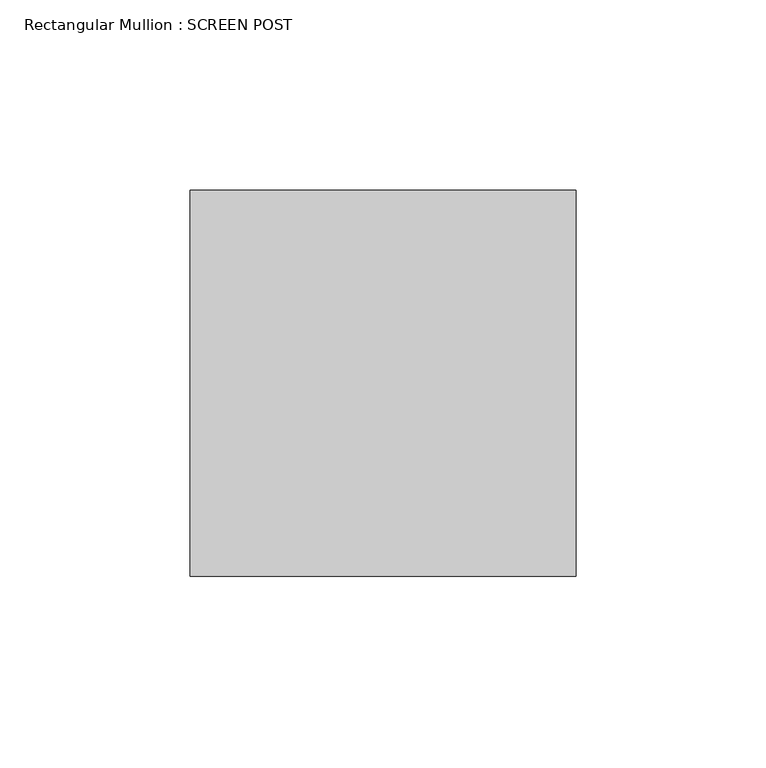
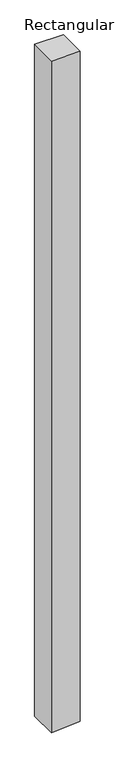
"""IFC4 building model written with IfcOpenShell, lengths in millimetres: member geometry, Rectangular Mullion : SCREEN POST."""

from ifc_helpers import new_model, si_unit, frame, origin, place, context, project, spatial, polyline, outline, extrude, source, transform, mapped, element, save


def rectangular_mullion_screen_post_556a0704(model_context):
    return source(origin(), model_context, "Body", "SweptSolid", [
        extrude(outline(polyline([(0.0, 50.8), (0.0, -50.8), (-2497.7934941, -50.8), (-2495.0102899, -6.3490391), (-2491.4320219, 50.8), (0.0, 50.8)])), frame((0.0, -50.8, 0.0), z_axis=(0.0, 1.0, 0.0), x_axis=(0.0, 0.0, 1.0)), (0.0, 0.0, 1.0), 101.6),
    ])


if __name__ == "__main__":
    model = new_model("IFC4")
    model_context = context("Model", 3, world=origin())
    ifc_project = project(units=[si_unit("LENGTHUNIT", "METRE", prefix="MILLI")], contexts=[model_context])
    site = spatial("IfcSite", under=ifc_project)
    building = spatial("IfcBuilding", under=site)
    placement = place(None, origin())
    rectangular_mullion_screen_post_shape = rectangular_mullion_screen_post_556a0704(model_context)
    element("IfcMember", 1, ObjectType="Rectangular Mullion : SCREEN POST", at=placement, inside=building, context=model_context, shape_type="MappedRepresentation", body=[
        mapped(rectangular_mullion_screen_post_shape, transform((0.0, 0.0, 0.0), x_axis=(1.0, 0.0, 0.0), y_axis=(0.0, 1.0, 0.0), z_axis=(0.0, 0.0, 1.0))),
    ])
    save(model, "model.ifc")

# Revit data of these elements
# Type "Rectangular Mullion : SCREEN POST"
#   built-in parameter 1007304 = 0.333333 (stored number, unit not read)
#   built-in parameter 1007301 = 0.166667 (stored number, unit not read)
#   built-in parameter 1007300 = 0.166667 (stored number, unit not read)
# Element 1 (IfcMember, "Rectangular Mullion : SCREEN POST")
#   Materials on its faces: "GLULAMS COLUMNS\n(PRESSURE TREATED W/ PENTA IN SOLVENT) (EXTERIOR STAIN: PENOFIN VERDE EXT. STAIN - COLOR: CEDAR)"
# Materials
#   "GLULAMS COLUMNS\n(PRESSURE TREATED W/ PENTA IN SOLVENT) (EXTERIOR STAIN: PENOFIN VERDE EXT. STAIN - COLOR: CEDAR)": class "Wood", colour RGB 164 134 123, transparency 0, Description = "Pinus Echinata", Cost = 0
